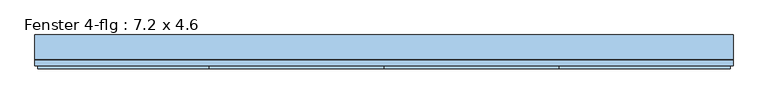
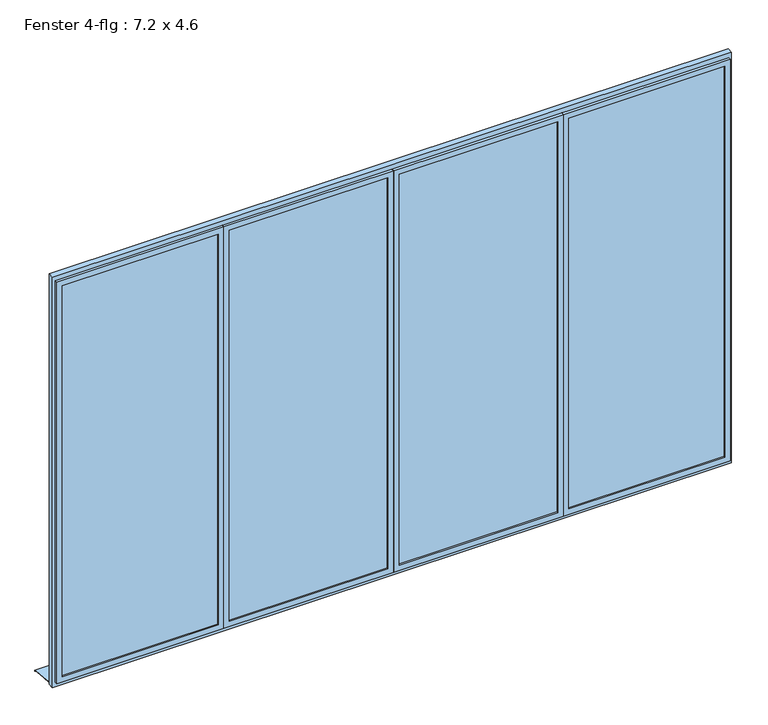
"""IFC4 building model written with IfcOpenShell, lengths in millimetres: window geometry, Fenster 4-flg : 7.2 x 4.6."""

from ifc_helpers import new_model, si_unit, frame, origin, place, context, project, spatial, polyline, outline, extrude, faceted_brep, source, transform, mapped, element, save


def fenster_4_flg_7_2_x_4_6_16c61e9f(model_context):
    return source(origin(), model_context, "Body", "SolidModel", [
        extrude(outline(polyline([(4300.0, 80.0), (4300.0, 20.0), (4240.0, 20.0), (4240.0, 80.0), (4300.0, 80.0)])), frame((0.0, 0.0, 1080.0), z_axis=(0.0, 0.0, 1.0), x_axis=(1.0, 0.0, 0.0)), (0.0, 0.0, 1.0), 4440.0),
        extrude(outline(polyline([(2500.0, 80.0), (2500.0, 20.0), (2440.0, 20.0), (2440.0, 80.0), (2500.0, 80.0)])), frame((0.0, 0.0, 1080.0), z_axis=(0.0, 0.0, 1.0), x_axis=(1.0, 0.0, 0.0)), (0.0, 0.0, 1.0), 4440.0),
        extrude(outline(polyline([(700.0, 80.0), (700.0, 20.0), (640.0, 20.0), (640.0, 80.0), (700.0, 80.0)])), frame((0.0, 0.0, 1080.0), z_axis=(0.0, 0.0, 1.0), x_axis=(1.0, 0.0, 0.0)), (0.0, 0.0, 1.0), 4440.0),
        extrude(outline(polyline([(5600.0, 6070.0), (5600.0, -1130.0), (1000.0, -1130.0), (1000.0, 6070.0), (5600.0, 6070.0)]), holes=[polyline([(5520.0, 6010.0), (1080.0, 6010.0), (1080.0, -1070.0), (5520.0, -1070.0), (5520.0, 6010.0)])]), frame((0.0, 20.0, 0.0), z_axis=(0.0, 1.0, 0.0), x_axis=(0.0, 0.0, 1.0)), (0.0, 0.0, 1.0), 60.0),
        faceted_brep([(4270.0, 20.0, 5550.0), (4270.0, -10.0, 5550.0), (4270.0, -10.0, 1050.0), (4270.0, 20.0, 1050.0), (2470.0, -10.0, 5550.0), (2470.0, -10.0, 1050.0), (4210.0, -10.0, 1110.0), (2530.0, -10.0, 1110.0), (2530.0, -10.0, 5490.0), (4210.0, -10.0, 5490.0), (2470.0, 20.0, 1050.0), (2470.0, 20.0, 5550.0), (4240.0, 20.0, 5520.0), (2500.0, 20.0, 5520.0), (2500.0, 20.0, 1080.0), (4240.0, 20.0, 1080.0), (4240.0, 50.0, 5520.0), (4240.0, 50.0, 1080.0), (2500.0, 50.0, 1080.0), (2500.0, 50.0, 5520.0), (4210.0, 50.0, 5490.0), (2530.0, 50.0, 5490.0), (2530.0, 50.0, 1110.0), (4210.0, 50.0, 1110.0)], [[[0, 1, 2, 3]], [[1, 4, 5, 2], [6, 7, 8, 9]], [[3, 2, 5, 10]], [[3, 10, 11, 0], [12, 13, 14, 15]], [[16, 12, 15, 17]], [[17, 15, 14, 18]], [[17, 18, 19, 16], [20, 21, 22, 23]], [[9, 20, 23, 6]], [[6, 23, 22, 7]], [[10, 5, 4, 11]], [[18, 14, 13, 19]], [[7, 22, 21, 8]], [[11, 4, 1, 0]], [[19, 13, 12, 16]], [[8, 21, 20, 9]]]),
        faceted_brep([(2470.0, 20.0, 5550.0), (2470.0, -10.0, 5550.0), (2470.0, -10.0, 1050.0), (2470.0, 20.0, 1050.0), (670.0, -10.0, 5550.0), (670.0, -10.0, 1050.0), (2410.0, -10.0, 1110.0), (730.0, -10.0, 1110.0), (730.0, -10.0, 5490.0), (2410.0, -10.0, 5490.0), (670.0, 20.0, 1050.0), (670.0, 20.0, 5550.0), (2440.0, 20.0, 5520.0), (700.0, 20.0, 5520.0), (700.0, 20.0, 1080.0), (2440.0, 20.0, 1080.0), (2440.0, 50.0, 5520.0), (2440.0, 50.0, 1080.0), (700.0, 50.0, 1080.0), (700.0, 50.0, 5520.0), (2410.0, 50.0, 5490.0), (730.0, 50.0, 5490.0), (730.0, 50.0, 1110.0), (2410.0, 50.0, 1110.0)], [[[0, 1, 2, 3]], [[1, 4, 5, 2], [6, 7, 8, 9]], [[3, 2, 5, 10]], [[3, 10, 11, 0], [12, 13, 14, 15]], [[16, 12, 15, 17]], [[17, 15, 14, 18]], [[17, 18, 19, 16], [20, 21, 22, 23]], [[9, 20, 23, 6]], [[6, 23, 22, 7]], [[10, 5, 4, 11]], [[18, 14, 13, 19]], [[7, 22, 21, 8]], [[11, 4, 1, 0]], [[19, 13, 12, 16]], [[8, 21, 20, 9]]]),
        faceted_brep([(670.0, 20.0, 5550.0), (670.0, -10.0, 5550.0), (670.0, -10.0, 1050.0), (670.0, 20.0, 1050.0), (-1100.0, -10.0, 5550.0), (-1100.0, -10.0, 1050.0), (610.0, -10.0, 1110.0), (-1040.0, -10.0, 1110.0), (-1040.0, -10.0, 5490.0), (610.0, -10.0, 5490.0), (-1100.0, 20.0, 1050.0), (-1100.0, 20.0, 5550.0), (640.0, 20.0, 5520.0), (-1070.0, 20.0, 5520.0), (-1070.0, 20.0, 1080.0), (640.0, 20.0, 1080.0), (640.0, 50.0, 5520.0), (640.0, 50.0, 1080.0), (-1070.0, 50.0, 1080.0), (-1070.0, 50.0, 5520.0), (610.0, 50.0, 5490.0), (-1040.0, 50.0, 5490.0), (-1040.0, 50.0, 1110.0), (610.0, 50.0, 1110.0)], [[[0, 1, 2, 3]], [[1, 4, 5, 2], [6, 7, 8, 9]], [[3, 2, 5, 10]], [[3, 10, 11, 0], [12, 13, 14, 15]], [[16, 12, 15, 17]], [[17, 15, 14, 18]], [[17, 18, 19, 16], [20, 21, 22, 23]], [[9, 20, 23, 6]], [[6, 23, 22, 7]], [[10, 5, 4, 11]], [[18, 14, 13, 19]], [[7, 22, 21, 8]], [[11, 4, 1, 0]], [[19, 13, 12, 16]], [[8, 21, 20, 9]]]),
        faceted_brep([(6040.0, 20.0, 5550.0), (6040.0, -10.0, 5550.0), (6040.0, -10.0, 1050.0), (6040.0, 20.0, 1050.0), (4270.0, -10.0, 5550.0), (4270.0, -10.0, 1050.0), (5980.0, -10.0, 1110.0), (4330.0, -10.0, 1110.0), (4330.0, -10.0, 5490.0), (5980.0, -10.0, 5490.0), (4270.0, 20.0, 1050.0), (4270.0, 20.0, 5550.0), (6010.0, 20.0, 5520.0), (4300.0, 20.0, 5520.0), (4300.0, 20.0, 1080.0), (6010.0, 20.0, 1080.0), (6010.0, 50.0, 5520.0), (6010.0, 50.0, 1080.0), (4300.0, 50.0, 1080.0), (4300.0, 50.0, 5520.0), (5980.0, 50.0, 5490.0), (4330.0, 50.0, 5490.0), (4330.0, 50.0, 1110.0), (5980.0, 50.0, 1110.0)], [[[0, 1, 2, 3]], [[1, 4, 5, 2], [6, 7, 8, 9]], [[3, 2, 5, 10]], [[3, 10, 11, 0], [12, 13, 14, 15]], [[16, 12, 15, 17]], [[17, 15, 14, 18]], [[17, 18, 19, 16], [20, 21, 22, 23]], [[9, 20, 23, 6]], [[6, 23, 22, 7]], [[10, 5, 4, 11]], [[18, 14, 13, 19]], [[7, 22, 21, 8]], [[11, 4, 1, 0]], [[19, 13, 12, 16]], [[8, 21, 20, 9]]]),
        extrude(outline(polyline([(90.0221543, 1020.0), (340.0, 1000.0), (340.0, 990.0), (338.0, 990.0), (338.0, 998.3604634), (89.8240723, 1018.0), (80.0, 1018.0), (80.0, 1020.0), (90.0221543, 1020.0)])), frame((-1130.0, 0.0, 0.0), z_axis=(1.0, 0.0, 0.0), x_axis=(0.0, 1.0, 0.0)), (0.0, 0.0, 1.0), 7200.0),
        extrude(outline(polyline([(610.0, 5.0), (-1040.0, 5.0), (-1040.0, 35.0), (610.0, 35.0), (610.0, 5.0)])), frame((0.0, 0.0, 1110.0), z_axis=(0.0, 0.0, 1.0), x_axis=(1.0, 0.0, 0.0)), (0.0, 0.0, 1.0), 4380.0),
        extrude(outline(polyline([(2410.0, 5.0), (730.0, 5.0), (730.0, 35.0), (2410.0, 35.0), (2410.0, 5.0)])), frame((0.0, 0.0, 1110.0), z_axis=(0.0, 0.0, 1.0), x_axis=(1.0, 0.0, 0.0)), (0.0, 0.0, 1.0), 4380.0),
        extrude(outline(polyline([(4210.0, 5.0), (2530.0, 5.0), (2530.0, 35.0), (4210.0, 35.0), (4210.0, 5.0)])), frame((0.0, 0.0, 1110.0), z_axis=(0.0, 0.0, 1.0), x_axis=(1.0, 0.0, 0.0)), (0.0, 0.0, 1.0), 4380.0),
        extrude(outline(polyline([(5980.0, 5.0), (4330.0, 5.0), (4330.0, 35.0), (5980.0, 35.0), (5980.0, 5.0)])), frame((0.0, 0.0, 1110.0), z_axis=(0.0, 0.0, 1.0), x_axis=(1.0, 0.0, 0.0)), (0.0, 0.0, 1.0), 4380.0),
    ])


if __name__ == "__main__":
    model = new_model("IFC4")
    model_context = context("Model", 3, world=origin())
    ifc_project = project(units=[si_unit("LENGTHUNIT", "METRE", prefix="MILLI")], contexts=[model_context])
    site = spatial("IfcSite", under=ifc_project)
    building = spatial("IfcBuilding", under=site)
    placement = place(None, origin())
    fenster_4_flg_7_2_x_4_6_shape = fenster_4_flg_7_2_x_4_6_16c61e9f(model_context)
    element("IfcWindow", 1, ObjectType="Fenster 4-flg : 7.2 x 4.6", at=placement, inside=building, context=model_context, shape_type="MappedRepresentation", body=[
        mapped(fenster_4_flg_7_2_x_4_6_shape, transform((0.0, 0.0, 0.0), x_axis=(1.0, 0.0, 0.0), y_axis=(0.0, 1.0, 0.0), z_axis=(0.0, 0.0, 1.0))),
    ])
    save(model, "model.ifc")

# Revit data of these elements
# Type "Fenster 4-flg : 7.2 x 4.6"
#   Type Mark = "55"
#   Operation = "UserDefined"
#   Keynote = "16.05.01"
#   Visual Light Transmittance = 0.9
#   Solar Heat Gain Coefficient = 0.78
#   Rough Height = 4.600 m
#   Rough Width = 7.200 m
#   Heat Transfer Coefficient (U) = 3.6886 W/(m²·K)
#   Rahmentiefe = 0.060 m
#   Breite unterer Rahmen = 0.080 m
#   Breite oberer  Rahmen = 0.080 m
#   Rahmenbreite = 0.060 m
#   Height = 4.600 m
#   Tiefe Flügel = 0.060 m
#   Flügelbreite = 0.060 m
#   Einbautiefe (von außen) [instance default] = 0.080 m
#   Width = 7.200 m
#   Bild = none
#   Glas = Fenster - Glas
#   Fensterflügel = Fenster - Kunststoff weiß
#   Innere Fensterbank = Fenster - Holz 1
#   Äußere Fensterbank = Fenster - Kunststoff weiß
#   Construction Type Id = ""
#   Wall Closure = (empty or 0)
#   Analytic Construction = (empty or 0)
# Element 1 (IfcWindow, "Fenster 4-flg : 7.2 x 4.6")
#   Einbautiefe (von außen) = 0.230 m
#   Materials on its faces: "Fenster - Kunststoff weiß", "Kunststoff - Weiß", "Fenster - Glas"
# Materials
#   "Fenster - Glas": class "Glas", colour RGB 128 128 255, transparency 0.75, Cost = 0
#   "Fenster - Kunststoff weiß": class "Kunststoff", colour RGB 249 249 249, transparency 0, Cost = 0
#   "Fenster - Holz 1": class "Holz", colour RGB 216 135 75, transparency 0, Cost = 0
#   "Kunststoff - Weiß": class "Kunststoff", colour RGB 249 249 249, transparency 0, Cost = 0
